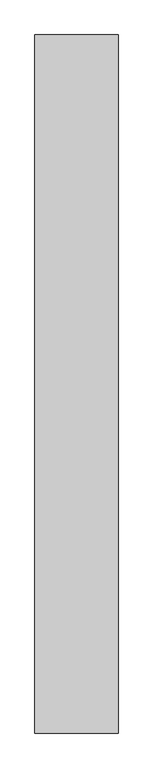
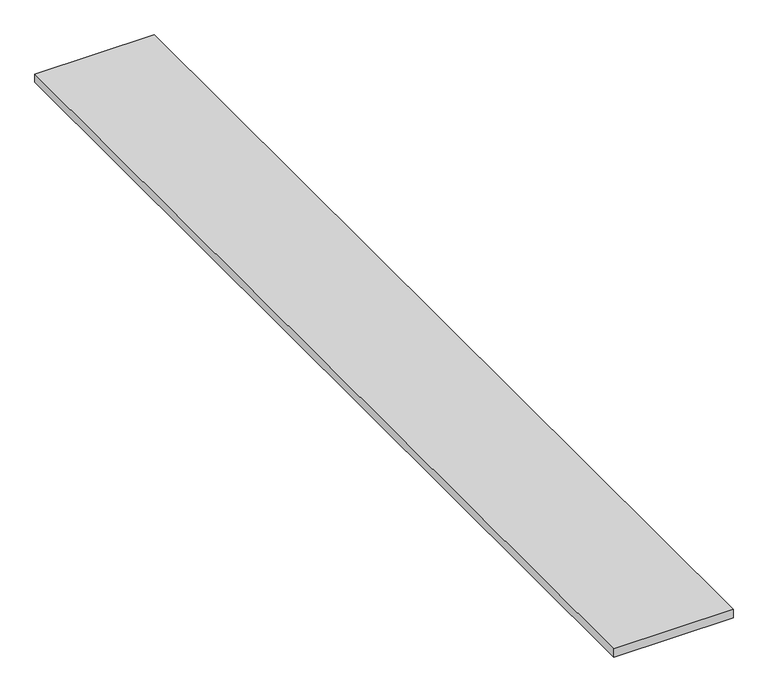
"""IFC4 building model written with IfcOpenShell, lengths in millimetres: furniture geometry, Furniture 1:Furniture 1:2341:Furniture 1:2341 : Furniture 1:Furniture 1:2341:300173 : Furniture 1:Furniture 1:2341:Furniture 1:2341 : Furniture 1:Furniture 1:2341:300173."""

from ifc_helpers import new_model, si_unit, frame, origin, place, context, project, spatial, polyline, outline, extrude, source, transform, mapped, element, save


def furniture_4c088013(model_context):
    return source(origin(), model_context, "Body", "SweptSolid", [
        extrude(outline(polyline([(651443.7117239, -575267.6690318), (651443.7117239, -572280.41257), (651799.3117239, -572280.41257), (651799.3117239, -575267.6690318), (651443.7117239, -575267.6690318)])), frame((0.0, 0.0, 381.0), z_axis=(0.0, 0.0, 1.0), x_axis=(1.0, 0.0, 0.0)), (0.0, 0.0, 1.0), 25.4),
    ])


if __name__ == "__main__":
    model = new_model("IFC4")
    model_context = context("Model", 3, world=origin())
    ifc_project = project(units=[si_unit("LENGTHUNIT", "METRE", prefix="MILLI")], contexts=[model_context])
    site = spatial("IfcSite", under=ifc_project)
    building = spatial("IfcBuilding", under=site)
    placement = place(None, origin())
    furniture_shape = furniture_4c088013(model_context)
    element("IfcFurniture", 1, ObjectType="Furniture 1:Furniture 1:2341:Furniture 1:2341 : Furniture 1:Furniture 1:2341:300173 : Furniture 1:Furniture 1:2341:Furniture 1:2341 : Furniture 1:Furniture 1:2341:300173", at=placement, inside=building, context=model_context, shape_type="MappedRepresentation", body=[
        mapped(furniture_shape, transform((0.0, 0.0, 0.0), x_axis=(1.0, 0.0, 0.0), y_axis=(0.0, 1.0, 0.0), z_axis=(0.0, 0.0, 1.0))),
    ])
    save(model, "model.ifc")

# Revit data of these elements
# Type "Furniture 1:Furniture 1:2341:Furniture 1:2341 : Furniture 1:Furniture 1:2341:300173 : Furniture 1:Furniture 1:2341:Furniture 1:2341 : Furniture 1:Furniture 1:2341:300173"
#   NameOverride = "Furniture 1:Furniture 1:2341:Furniture 1:2341 : Furniture 1:Furniture 1:2341:300173"
#   ObjectTypeOverride = "Furniture 1:2341 : Furniture 1:Furniture 1:2341"
#   Tag = "300173"
